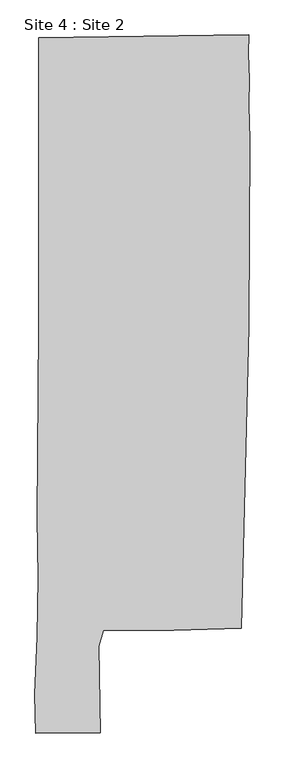
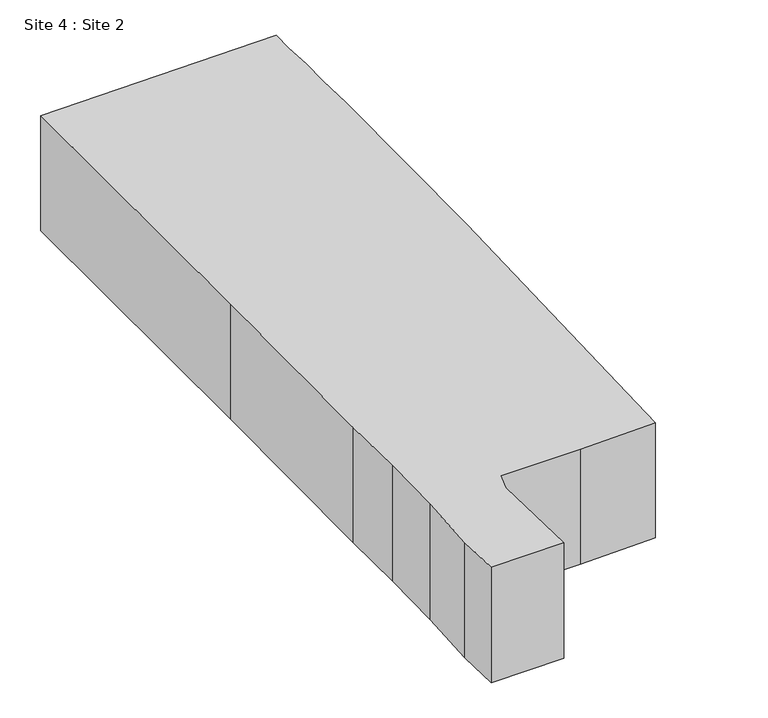
"""IFC4 building model written with IfcOpenShell, lengths in millimetres: geographic element geometry, Site 4 : Site 2."""

from ifc_helpers import new_model, si_unit, frame, origin, place, context, project, spatial, polyline, outline, extrude, source, transform, mapped, element, save


def site_4_site_2_d3c7b1b5(model_context):
    return source(origin(), model_context, "Body", "SweptSolid", [
        extrude(outline(polyline([(47069.739469, 118051.0435782), (47043.2485504, 116222.4753159), (47109.5144512, 113782.9125819), (47019.7812823, 100575.0298085), (46507.5402416, 79244.5499285), (41729.8960793, 79110.547942), (36750.5493833, 79081.0765167), (36429.590646, 77968.03341), (36544.4654549, 71869.8200444), (31971.4757273, 71834.4616257), (31909.6213599, 74578.828126), (32070.0814264, 78640.8413742), (32130.4224653, 82805.9558551), (32090.6432502, 87074.0869127), (32183.3240873, 100485.1438761), (32175.8424465, 121010.2431952), (47013.7719724, 121201.7585813), (46994.6390291, 119881.0836194), (47069.739469, 118051.0435782)])), frame((0.0, 0.0, 266395.2), z_axis=(0.0, 0.0, 1.0), x_axis=(1.0, 0.0, 0.0)), (0.0, 0.0, 1.0), 7620.0),
    ])


if __name__ == "__main__":
    model = new_model("IFC4")
    model_context = context("Model", 3, world=origin())
    ifc_project = project(units=[si_unit("LENGTHUNIT", "METRE", prefix="MILLI")], contexts=[model_context])
    site = spatial("IfcSite", under=ifc_project)
    building = spatial("IfcBuilding", under=site)
    placement = place(None, origin())
    site_4_site_2_shape = site_4_site_2_d3c7b1b5(model_context)
    element("IfcGeographicElement", 1, ObjectType="Site 4 : Site 2", at=placement, inside=building, context=model_context, shape_type="MappedRepresentation", body=[
        mapped(site_4_site_2_shape, transform((0.0, 0.0, 0.0), x_axis=(1.0, 0.0, 0.0), y_axis=(0.0, 1.0, 0.0), z_axis=(0.0, 0.0, 1.0))),
    ])
    save(model, "model.ifc")

# Revit data of these elements
# Element 1 (IfcGeographicElement, "Site 4 : Site 2")
#   Materials on its faces: "EXISTING BUILDING"
# Materials
#   "EXISTING BUILDING": class "Generic", colour RGB 120 120 120, transparency 0, Cost = 0
